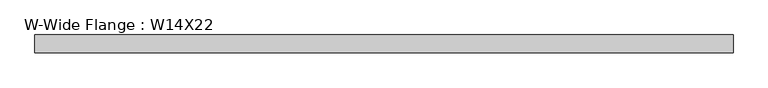
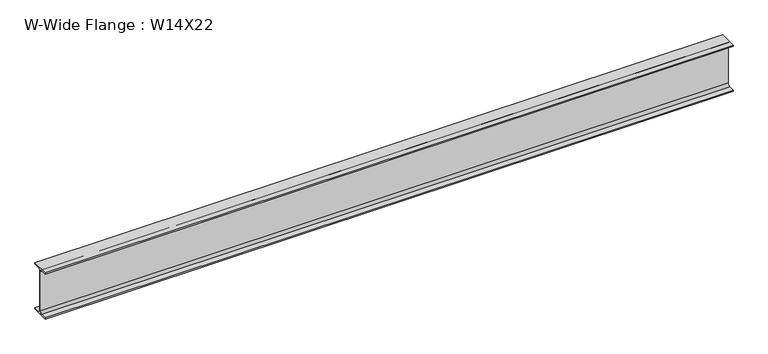
"""IFC4 building model written with IfcOpenShell, lengths in millimetres: beam geometry, W-Wide Flange : W14X22."""

from ifc_helpers import new_model, si_unit, point, frame, frame_2d, origin, place, context, project, spatial, polyline, circle_curve, trimmed, segment, composite_curve, outline, extrude, source, transform, mapped, element, save


def w_wide_flange_w14x22_59cbeafc(model_context):
    return source(origin(), model_context, "Body", "SweptSolid", [
        extrude(outline(composite_curve([segment(polyline([(63.5, -165.481), (63.5, -173.99), (-63.5, -173.99), (-63.5, -165.481), (-21.3995, -165.481)]), True, "CONTINUOUS"), segment(trimmed(circle_curve(frame_2d((-21.3995, -147.0025)), 18.4785), [point((-21.3995, -165.481))], [point((-2.921, -147.0025))], True, "CARTESIAN"), True, "CONTINUOUS"), segment(polyline([(-2.921, -147.0025), (-2.921, 147.0025)]), True, "CONTINUOUS"), segment(trimmed(circle_curve(frame_2d((-21.3995, 147.0025)), 18.4785), [point((-2.921, 147.0025))], [point((-21.3995, 165.481))], True, "CARTESIAN"), True, "CONTINUOUS"), segment(polyline([(-21.3995, 165.481), (-63.5, 165.481), (-63.5, 173.99), (63.5, 173.99), (63.5, 165.481), (21.3995, 165.481)]), True, "CONTINUOUS"), segment(trimmed(circle_curve(frame_2d((21.3995, 147.0025)), 18.4785), [point((21.3995, 165.481))], [point((2.921, 147.0025))], True, "CARTESIAN"), True, "CONTINUOUS"), segment(polyline([(2.921, 147.0025), (2.921, -147.0025)]), True, "CONTINUOUS"), segment(trimmed(circle_curve(frame_2d((21.3995, -147.0025)), 18.4785), [point((2.921, -147.0025))], [point((21.3995, -165.481))], True, "CARTESIAN"), True, "CONTINUOUS"), segment(polyline([(21.3995, -165.481), (63.5, -165.481)]), True, "CONTINUOUS")], self_intersect=False)), frame((-2429.0183341, 0.0, 0.0), z_axis=(1.0, 0.0, 0.0), x_axis=(0.0, 1.0, 0.0)), (0.0, 0.0, 1.0), 4912.4195312),
    ])


if __name__ == "__main__":
    model = new_model("IFC4")
    model_context = context("Model", 3, world=origin())
    ifc_project = project(units=[si_unit("LENGTHUNIT", "METRE", prefix="MILLI")], contexts=[model_context])
    site = spatial("IfcSite", under=ifc_project)
    building = spatial("IfcBuilding", under=site)
    placement = place(None, origin())
    w_wide_flange_w14x22_shape = w_wide_flange_w14x22_59cbeafc(model_context)
    element("IfcBeam", 1, ObjectType="W-Wide Flange : W14X22", at=placement, inside=building, context=model_context, shape_type="MappedRepresentation", body=[
        mapped(w_wide_flange_w14x22_shape, transform((0.0, 0.0, 0.0), x_axis=(1.0, 0.0, 0.0), y_axis=(0.0, 1.0, 0.0), z_axis=(0.0, 0.0, 1.0))),
    ])
    save(model, "model.ifc")

# Revit data of these elements
# Type "W-Wide Flange : W14X22"
#   Assembly Code = "B10"
#   W = 22
#   Length [instance default] = 1524 mm
#   bf = 127 mm
#   d = 347.98 mm
#   k = 26.988 mm
#   k2 = 18.479 mm
#   tf = 8.509 mm
#   tw = 5.842 mm
#   A = 0.00418709 m²
#   Structural Material [instance default] = Steel ASTM A992
# Element 1 (IfcBeam, "W-Wide Flange : W14X22")
#   Structural Material = Aluminum, Anodized Red
#   Materials on its faces: "Aluminum, Anodized Red"
# Materials
#   "Steel ASTM A992": class "Metal", colour RGB 128 0 0, transparency 0, Description = "Structural steel 50ksi", Cost = 0
#   "Aluminum, Anodized Red": class "Metal", colour RGB 120 120 120, transparency 0, Description = "Anodized aluminum, red", Cost = 0
